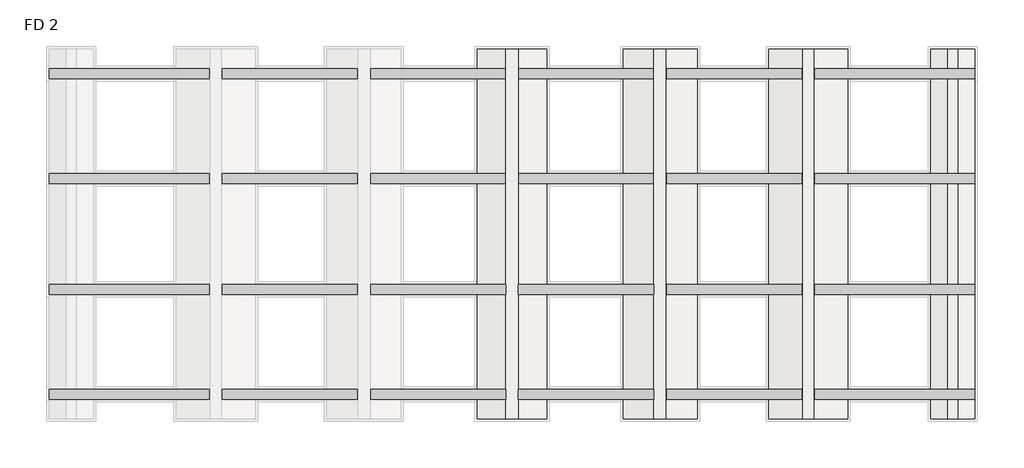
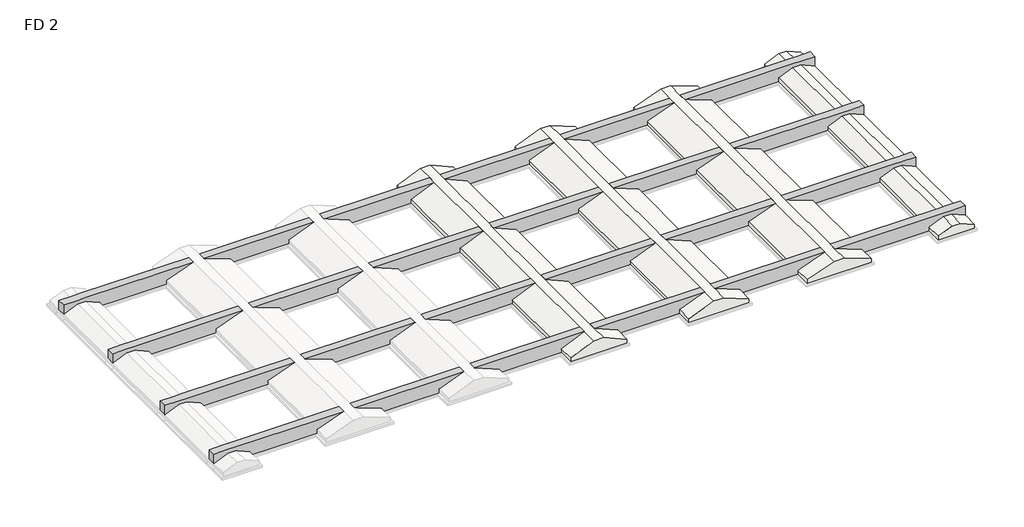
# One storey, part 2 of 2: 4 beams, 4 slabs.
"""IFC4 building model written with IfcOpenShell, lengths in millimetres."""

from ifc_helpers import new_model, si_unit, origin, place, context, project, spatial, faceted_brep, element, save

model = new_model("IFC4")

# Units and contexts
model_context = context("Model", 3, world=origin())
ifc_project = project(units=[si_unit("LENGTHUNIT", "METRE", prefix="MILLI")], contexts=[model_context])

# Site, building, storey
site = spatial("IfcSite", under=ifc_project)
building = spatial("IfcBuilding", under=site)
storey = spatial("IfcBuildingStorey", under=building, Name="FD 2", Elevation=-2170.0)

# Beams
placement = place(None, origin())
element("IfcBeam", 1, ObjectType="M_Concrete-Rectangular Beam : 400x700", at=placement, inside=storey, context=model_context, shape_type="Brep", body=[
    faceted_brep([(-900.0, 12800.0000002, -1470.0), (-900.0, 13200.0000002, -1470.0), (-900.0, 13200.0000002, -1970.0), (-900.0, 12800.0000002, -1970.0), (-200.0, 12800.0000002, -1470.0), (200.0, 12800.0000002, -1470.0), (5600.0000012, 12800.0000002, -1470.0), (5600.0000012, 13200.0000002, -1470.0), (200.0, 13200.0000002, -1470.0), (-200.0, 13200.0000002, -1470.0), (4250.0000012, 13200.0000002, -1970.0), (4250.0000012, 13200.0000002, -2170.0), (900.0, 13200.0000002, -2170.0), (900.0, 13200.0000002, -1970.0), (200.0, 13200.0000002, -1670.0), (-200.0, 13200.0000002, -1670.0), (900.0, 12800.0000002, -2170.0), (4250.0000012, 12800.0000002, -2170.0), (-200.0, 12800.0000002, -1670.0), (200.0, 12800.0000002, -1670.0), (900.0, 12800.0000002, -1970.0), (4250.0000012, 12800.0000002, -1970.0)], [[[0, 1, 2, 3]], [[1, 0, 4, 5, 6, 7, 8, 9]], [[2, 1, 9, 8, 7, 10, 11, 12, 13, 14, 15]], [[16, 12, 11, 17]], [[0, 3, 18, 19, 20, 16, 17, 21, 6, 5, 4]], [[20, 13, 12, 16]], [[13, 20, 19, 14]], [[15, 14, 19, 18]], [[21, 10, 7, 6]], [[10, 21, 17, 11]], [[3, 2, 15, 18]]]),
    faceted_brep([(36599.948043, 13200.0000002, -1470.0), (36599.948043, 12800.0000002, -1470.0), (36599.948043, 12800.0000002, -1970.0), (36599.948043, 13200.0000002, -1970.0), (35899.948043, 12800.0000002, -1670.0), (35899.948043, 13200.0000002, -1670.0), (34799.948043, 13200.0000002, -1970.0), (34799.948043, 12800.0000002, -1970.0), (34799.948043, 12800.0000002, -2170.0), (34799.948043, 13200.0000002, -2170.0), (35499.948043, 13200.0000002, -1670.0), (35499.948043, 12800.0000002, -1670.0), (31449.9130271, 12800.0000002, -1970.0), (31449.9130271, 13200.0000002, -1970.0), (31449.9130271, 13200.0000002, -2170.0), (31449.9130271, 12800.0000002, -2170.0), (30099.9130271, 12800.0000002, -1470.0), (30099.9130271, 13200.0000002, -1470.0), (35899.948043, 13200.0000002, -1470.0), (35499.948043, 13200.0000002, -1470.0), (35499.948043, 12800.0000002, -1470.0), (35899.948043, 12800.0000002, -1470.0)], [[[0, 1, 2, 3]], [[3, 2, 4, 5]], [[6, 7, 8, 9]], [[7, 6, 10, 11]], [[5, 4, 11, 10]], [[12, 13, 14, 15]], [[13, 12, 16, 17]], [[9, 8, 15, 14]], [[1, 0, 18, 19, 17, 16, 20, 21]], [[0, 3, 5, 10, 6, 9, 14, 13, 17, 19, 18]], [[2, 1, 21, 20, 16, 12, 15, 8, 7, 11, 4]]]),
    faceted_brep([(7450.0000012, 12800.0000002, -1970.0), (7450.0000012, 13200.0000002, -1970.0), (7450.0000012, 13200.0000002, -2170.0), (7450.0000012, 12800.0000002, -2170.0), (6100.0000012, 12800.0000002, -1470.0), (6100.0000012, 13200.0000002, -1470.0), (10349.9130239, 13200.0000002, -2170.0), (10349.9130239, 12800.0000002, -2170.0), (10349.9130239, 12800.0000002, -1970.0), (10349.9130239, 13200.0000002, -1970.0), (11599.9130239, 13200.0000002, -1470.0), (11599.9130239, 12800.0000002, -1470.0)], [[[0, 1, 2, 3]], [[1, 0, 4, 5]], [[3, 2, 6, 7]], [[8, 9, 10, 11]], [[9, 8, 7, 6]], [[5, 4, 11, 10]], [[2, 1, 5, 10, 9, 6]], [[3, 7, 8, 11, 4, 0]]]),
    faceted_brep([(13349.9130239, 12800.0000002, -1970.0), (13349.9130239, 13200.0000002, -1970.0), (13349.9130239, 13200.0000002, -2170.0), (13349.9130239, 12800.0000002, -2170.0), (12099.9130239, 12800.0000002, -1470.0), (12099.9130239, 13200.0000002, -1470.0), (16449.7667691, 13200.0000002, -2170.0), (16449.7667691, 12800.0000002, -2170.0), (16449.7667691, 12800.0000002, -1970.0), (16449.7667691, 13200.0000002, -1970.0), (17599.7667691, 13200.0000002, -1470.0), (17599.7667691, 12800.0000002, -1470.0)], [[[0, 1, 2, 3]], [[1, 0, 4, 5]], [[3, 2, 6, 7]], [[8, 9, 10, 11]], [[9, 8, 7, 6]], [[5, 4, 11, 10]], [[2, 1, 5, 10, 9, 6]], [[3, 7, 8, 11, 4, 0]]]),
    faceted_brep([(19249.7667691, 12800.0000002, -1970.0), (19249.7667691, 13200.0000002, -1970.0), (19249.7667691, 13200.0000002, -2170.0), (19249.7667691, 12800.0000002, -2170.0), (18099.7667691, 12800.0000002, -1470.0), (18099.7667691, 13200.0000002, -1470.0), (22349.9130289, 13200.0000002, -2170.0), (22349.9130289, 12800.0000002, -2170.0), (22349.9130289, 12800.0000002, -1970.0), (22349.9130289, 13200.0000002, -1970.0), (23599.9130289, 13200.0000002, -1470.0), (23599.9130289, 12800.0000002, -1470.0)], [[[0, 1, 2, 3]], [[1, 0, 4, 5]], [[3, 2, 6, 7]], [[8, 9, 10, 11]], [[9, 8, 7, 6]], [[5, 4, 11, 10]], [[2, 1, 5, 10, 9, 6]], [[3, 7, 8, 11, 4, 0]]]),
    faceted_brep([(25349.9130289, 12800.0000002, -1970.0), (25349.9130289, 13200.0000002, -1970.0), (25349.9130289, 13200.0000002, -2170.0), (25349.9130289, 12800.0000002, -2170.0), (24099.9130289, 12800.0000002, -1470.0), (24099.9130289, 13200.0000002, -1470.0), (28249.9130271, 13200.0000002, -2170.0), (28249.9130271, 12800.0000002, -2170.0), (28249.9130271, 12800.0000002, -1970.0), (28249.9130271, 13200.0000002, -1970.0), (29599.9130271, 13200.0000002, -1470.0), (29599.9130271, 12800.0000002, -1470.0)], [[[0, 1, 2, 3]], [[1, 0, 4, 5]], [[3, 2, 6, 7]], [[8, 9, 10, 11]], [[9, 8, 7, 6]], [[5, 4, 11, 10]], [[2, 1, 5, 10, 9, 6]], [[0, 3, 7, 8, 11, 4]]]),
])
element("IfcBeam", 2, ObjectType="M_Concrete-Rectangular Beam : 400x700", at=placement, inside=storey, context=model_context, shape_type="Brep", body=[
    faceted_brep([(-900.0, 8550.0000002, -1470.0), (-900.0, 8950.0000002, -1470.0), (-900.0, 8950.0000002, -1970.0), (-900.0, 8550.0000002, -1970.0), (-200.0, 8550.0000002, -1470.0), (200.0, 8550.0000002, -1470.0), (5600.0000012, 8550.0000002, -1470.0), (5600.0000012, 8950.0000002, -1470.0), (200.0, 8950.0000002, -1470.0), (-200.0, 8950.0000002, -1470.0), (4250.0000012, 8950.0000002, -1970.0), (4250.0000012, 8950.0000002, -2170.0), (900.0, 8950.0000002, -2170.0), (900.0, 8950.0000002, -1970.0), (200.0, 8950.0000002, -1670.0), (-200.0, 8950.0000002, -1670.0), (900.0, 8550.0000002, -2170.0), (4250.0000012, 8550.0000002, -2170.0), (-200.0, 8550.0000002, -1670.0), (200.0, 8550.0000002, -1670.0), (900.0, 8550.0000002, -1970.0), (4250.0000012, 8550.0000002, -1970.0)], [[[0, 1, 2, 3]], [[1, 0, 4, 5, 6, 7, 8, 9]], [[2, 1, 9, 8, 7, 10, 11, 12, 13, 14, 15]], [[16, 12, 11, 17]], [[0, 3, 18, 19, 20, 16, 17, 21, 6, 5, 4]], [[3, 2, 15, 18]], [[20, 13, 12, 16]], [[13, 20, 19, 14]], [[15, 14, 19, 18]], [[21, 10, 7, 6]], [[10, 21, 17, 11]]]),
    faceted_brep([(36599.948043, 8950.0000002, -1470.0), (36599.948043, 8550.0000002, -1470.0), (36599.948043, 8550.0000002, -1970.0), (36599.948043, 8950.0000002, -1970.0), (35899.948043, 8550.0000002, -1670.0), (35899.948043, 8950.0000002, -1670.0), (34799.948043, 8950.0000002, -1970.0), (34799.948043, 8550.0000002, -1970.0), (34799.948043, 8550.0000002, -2170.0), (34799.948043, 8950.0000002, -2170.0), (35499.948043, 8950.0000002, -1670.0), (35499.948043, 8550.0000002, -1670.0), (31449.9130271, 8550.0000002, -1970.0), (31449.9130271, 8950.0000002, -1970.0), (31449.9130271, 8950.0000002, -2170.0), (31449.9130271, 8550.0000002, -2170.0), (30099.9130271, 8550.0000002, -1470.0), (30099.9130271, 8950.0000002, -1470.0), (35899.948043, 8950.0000002, -1470.0), (35499.948043, 8950.0000002, -1470.0), (35499.948043, 8550.0000002, -1470.0), (35899.948043, 8550.0000002, -1470.0)], [[[0, 1, 2, 3]], [[3, 2, 4, 5]], [[6, 7, 8, 9]], [[7, 6, 10, 11]], [[5, 4, 11, 10]], [[12, 13, 14, 15]], [[13, 12, 16, 17]], [[9, 8, 15, 14]], [[1, 0, 18, 19, 17, 16, 20, 21]], [[0, 3, 5, 10, 6, 9, 14, 13, 17, 19, 18]], [[2, 1, 21, 20, 16, 12, 15, 8, 7, 11, 4]]]),
    faceted_brep([(7450.0000012, 8550.0000002, -1970.0), (7450.0000012, 8950.0000002, -1970.0), (7450.0000012, 8950.0000002, -2170.0), (7450.0000012, 8550.0000002, -2170.0), (6100.0000012, 8550.0000002, -1470.0), (6100.0000012, 8950.0000002, -1470.0), (10349.9130239, 8950.0000002, -2170.0), (10349.9130239, 8550.0000002, -2170.0), (10349.9130239, 8550.0000002, -1970.0), (10349.9130239, 8950.0000002, -1970.0), (11599.9130239, 8950.0000002, -1470.0), (11599.9130239, 8550.0000002, -1470.0)], [[[0, 1, 2, 3]], [[1, 0, 4, 5]], [[3, 2, 6, 7]], [[8, 9, 10, 11]], [[9, 8, 7, 6]], [[5, 4, 11, 10]], [[2, 1, 5, 10, 9, 6]], [[3, 7, 8, 11, 4, 0]]]),
    faceted_brep([(13349.9130239, 8550.0000002, -1970.0), (13349.9130239, 8950.0000002, -1970.0), (13349.9130239, 8950.0000002, -2170.0), (13349.9130239, 8550.0000002, -2170.0), (12099.9130239, 8550.0000002, -1470.0), (12099.9130239, 8950.0000002, -1470.0), (16449.7667691, 8950.0000002, -2170.0), (16449.7667691, 8550.0000002, -2170.0), (16449.7667691, 8550.0000002, -1970.0), (16449.7667691, 8950.0000002, -1970.0), (17599.7667691, 8950.0000002, -1470.0), (17599.7667691, 8550.0000002, -1470.0)], [[[0, 1, 2, 3]], [[1, 0, 4, 5]], [[3, 2, 6, 7]], [[8, 9, 10, 11]], [[9, 8, 7, 6]], [[5, 4, 11, 10]], [[2, 1, 5, 10, 9, 6]], [[3, 7, 8, 11, 4, 0]]]),
    faceted_brep([(19249.7667691, 8550.0000002, -1970.0), (19249.7667691, 8950.0000002, -1970.0), (19249.7667691, 8950.0000002, -2170.0), (19249.7667691, 8550.0000002, -2170.0), (18099.7667691, 8550.0000002, -1470.0), (18099.7667691, 8950.0000002, -1470.0), (22349.9130289, 8950.0000002, -2170.0), (22349.9130289, 8550.0000002, -2170.0), (22349.9130289, 8550.0000002, -1970.0), (22349.9130289, 8950.0000002, -1970.0), (23599.9130289, 8950.0000002, -1470.0), (23599.9130289, 8550.0000002, -1470.0)], [[[0, 1, 2, 3]], [[1, 0, 4, 5]], [[3, 2, 6, 7]], [[8, 9, 10, 11]], [[9, 8, 7, 6]], [[5, 4, 11, 10]], [[2, 1, 5, 10, 9, 6]], [[3, 7, 8, 11, 4, 0]]]),
    faceted_brep([(25349.9130289, 8550.0000002, -1970.0), (25349.9130289, 8950.0000002, -1970.0), (25349.9130289, 8950.0000002, -2170.0), (25349.9130289, 8550.0000002, -2170.0), (24099.9130289, 8550.0000002, -1470.0), (24099.9130289, 8950.0000002, -1470.0), (28249.9130271, 8950.0000002, -2170.0), (28249.9130271, 8550.0000002, -2170.0), (28249.9130271, 8550.0000002, -1970.0), (28249.9130271, 8950.0000002, -1970.0), (29599.9130271, 8950.0000002, -1470.0), (29599.9130271, 8550.0000002, -1470.0)], [[[0, 1, 2, 3]], [[1, 0, 4, 5]], [[3, 2, 6, 7]], [[8, 9, 10, 11]], [[9, 8, 7, 6]], [[5, 4, 11, 10]], [[2, 1, 5, 10, 9, 6]], [[0, 3, 7, 8, 11, 4]]]),
])
element("IfcBeam", 3, ObjectType="M_Concrete-Rectangular Beam : 400x700", at=placement, inside=storey, context=model_context, shape_type="Brep", body=[
    faceted_brep([(-900.0, 4050.0000002, -1470.0), (-900.0, 4450.0000002, -1470.0), (-900.0, 4450.0000002, -1970.0), (-900.0, 4050.0000002, -1970.0), (-200.0, 4050.0000002, -1470.0), (200.0, 4050.0000002, -1470.0), (5600.0000012, 4050.0000002, -1470.0), (5600.0000012, 4450.0000002, -1470.0), (200.0, 4450.0000002, -1470.0), (-200.0, 4450.0000002, -1470.0), (4250.0000012, 4450.0000002, -1970.0), (4250.0000012, 4450.0000002, -2170.0), (900.0, 4450.0000002, -2170.0), (900.0, 4450.0000002, -1970.0), (200.0, 4450.0000002, -1670.0), (-200.0, 4450.0000002, -1670.0), (900.0, 4050.0000002, -2170.0), (4250.0000012, 4050.0000002, -2170.0), (-200.0, 4050.0000002, -1670.0), (200.0, 4050.0000002, -1670.0), (900.0, 4050.0000002, -1970.0), (4250.0000012, 4050.0000002, -1970.0)], [[[0, 1, 2, 3]], [[1, 0, 4, 5, 6, 7, 8, 9]], [[2, 1, 9, 8, 7, 10, 11, 12, 13, 14, 15]], [[16, 12, 11, 17]], [[0, 3, 18, 19, 20, 16, 17, 21, 6, 5, 4]], [[3, 2, 15, 18]], [[20, 13, 12, 16]], [[13, 20, 19, 14]], [[15, 14, 19, 18]], [[21, 10, 7, 6]], [[10, 21, 17, 11]]]),
    faceted_brep([(36599.948043, 4450.0000002, -1470.0), (36599.948043, 4050.0000002, -1470.0), (36599.948043, 4050.0000002, -1970.0), (36599.948043, 4450.0000002, -1970.0), (35899.948043, 4050.0000002, -1670.0), (35899.948043, 4450.0000002, -1670.0), (34799.948043, 4450.0000002, -1970.0), (34799.948043, 4050.0000002, -1970.0), (34799.948043, 4050.0000002, -2170.0), (34799.948043, 4450.0000002, -2170.0), (35499.948043, 4450.0000002, -1670.0), (35499.948043, 4050.0000002, -1670.0), (31449.9130271, 4050.0000002, -1970.0), (31449.9130271, 4450.0000002, -1970.0), (31449.9130271, 4450.0000002, -2170.0), (31449.9130271, 4050.0000002, -2170.0), (30099.9130271, 4050.0000002, -1470.0), (30099.9130271, 4450.0000002, -1470.0), (35899.948043, 4450.0000002, -1470.0), (35499.948043, 4450.0000002, -1470.0), (35499.948043, 4050.0000002, -1470.0), (35899.948043, 4050.0000002, -1470.0)], [[[0, 1, 2, 3]], [[3, 2, 4, 5]], [[6, 7, 8, 9]], [[7, 6, 10, 11]], [[5, 4, 11, 10]], [[12, 13, 14, 15]], [[13, 12, 16, 17]], [[9, 8, 15, 14]], [[1, 0, 18, 19, 17, 16, 20, 21]], [[0, 3, 5, 10, 6, 9, 14, 13, 17, 19, 18]], [[2, 1, 21, 20, 16, 12, 15, 8, 7, 11, 4]]]),
    faceted_brep([(7450.0000012, 4050.0000002, -1970.0), (7450.0000012, 4450.0000002, -1970.0), (7450.0000012, 4450.0000002, -2170.0), (7450.0000012, 4050.0000002, -2170.0), (6100.0000012, 4050.0000002, -1470.0), (6100.0000012, 4450.0000002, -1470.0), (10349.9130239, 4450.0000002, -2170.0), (10349.9130239, 4050.0000002, -2170.0), (10349.9130239, 4050.0000002, -1970.0), (10349.9130239, 4450.0000002, -1970.0), (11599.9130239, 4450.0000002, -1470.0), (11599.9130239, 4050.0000002, -1470.0)], [[[0, 1, 2, 3]], [[1, 0, 4, 5]], [[3, 2, 6, 7]], [[8, 9, 10, 11]], [[9, 8, 7, 6]], [[5, 4, 11, 10]], [[2, 1, 5, 10, 9, 6]], [[3, 7, 8, 11, 4, 0]]]),
    faceted_brep([(13349.9130239, 4050.0000002, -1970.0), (13349.9130239, 4450.0000002, -1970.0), (13349.9130239, 4450.0000002, -2170.0), (13349.9130239, 4050.0000002, -2170.0), (12099.9130239, 4050.0000002, -1470.0), (12099.9130239, 4450.0000002, -1470.0), (16449.7667691, 4450.0000002, -2170.0), (16449.7667691, 4050.0000002, -2170.0), (16449.7667691, 4050.0000002, -1970.0), (16449.7667691, 4450.0000002, -1970.0), (17599.7667691, 4450.0000002, -1470.0), (17599.7667691, 4050.0000002, -1470.0)], [[[0, 1, 2, 3]], [[1, 0, 4, 5]], [[3, 2, 6, 7]], [[8, 9, 10, 11]], [[9, 8, 7, 6]], [[5, 4, 11, 10]], [[2, 1, 5, 10, 9, 6]], [[3, 7, 8, 11, 4, 0]]]),
    faceted_brep([(19249.7667691, 4050.0000002, -1970.0), (19249.7667691, 4450.0000002, -1970.0), (19249.7667691, 4450.0000002, -2170.0), (19249.7667691, 4050.0000002, -2170.0), (18099.7667691, 4050.0000002, -1470.0), (18099.7667691, 4450.0000002, -1470.0), (22349.9130289, 4450.0000002, -2170.0), (22349.9130289, 4050.0000002, -2170.0), (22349.9130289, 4050.0000002, -1970.0), (22349.9130289, 4450.0000002, -1970.0), (23599.9130289, 4450.0000002, -1470.0), (23599.9130289, 4050.0000002, -1470.0)], [[[0, 1, 2, 3]], [[1, 0, 4, 5]], [[3, 2, 6, 7]], [[8, 9, 10, 11]], [[9, 8, 7, 6]], [[5, 4, 11, 10]], [[2, 1, 5, 10, 9, 6]], [[3, 7, 8, 11, 4, 0]]]),
    faceted_brep([(25349.9130289, 4050.0000002, -1970.0), (25349.9130289, 4450.0000002, -1970.0), (25349.9130289, 4450.0000002, -2170.0), (25349.9130289, 4050.0000002, -2170.0), (24099.9130289, 4050.0000002, -1470.0), (24099.9130289, 4450.0000002, -1470.0), (28249.9130271, 4450.0000002, -2170.0), (28249.9130271, 4050.0000002, -2170.0), (28249.9130271, 4050.0000002, -1970.0), (28249.9130271, 4450.0000002, -1970.0), (29599.9130271, 4450.0000002, -1470.0), (29599.9130271, 4050.0000002, -1470.0)], [[[0, 1, 2, 3]], [[1, 0, 4, 5]], [[3, 2, 6, 7]], [[8, 9, 10, 11]], [[9, 8, 7, 6]], [[5, 4, 11, 10]], [[2, 1, 5, 10, 9, 6]], [[0, 3, 7, 8, 11, 4]]]),
])
element("IfcBeam", 4, ObjectType="M_Concrete-Rectangular Beam : 400x700", at=placement, inside=storey, context=model_context, shape_type="Brep", body=[
    faceted_brep([(-900.0, -200.0, -1470.0), (-900.0, 200.0, -1470.0), (-900.0, 200.0, -1970.0), (-900.0, -200.0, -1970.0), (-200.0, -200.0, -1470.0), (200.0, -200.0, -1470.0), (5600.0000012, -200.0, -1470.0), (5600.0000012, 200.0, -1470.0), (200.0, 200.0, -1470.0), (-200.0, 200.0, -1470.0), (4250.0000012, 200.0, -1970.0), (4250.0000012, 200.0, -2170.0), (900.0, 200.0, -2170.0), (900.0, 200.0, -1970.0), (200.0, 200.0, -1670.0), (-200.0, 200.0, -1670.0), (900.0, -200.0, -2170.0), (4250.0000012, -200.0, -2170.0), (-200.0, -200.0, -1670.0), (200.0, -200.0, -1670.0), (900.0, -200.0, -1970.0), (4250.0000012, -200.0, -1970.0)], [[[0, 1, 2, 3]], [[1, 0, 4, 5, 6, 7, 8, 9]], [[2, 1, 9, 8, 7, 10, 11, 12, 13, 14, 15]], [[16, 12, 11, 17]], [[0, 3, 18, 19, 20, 16, 17, 21, 6, 5, 4]], [[3, 2, 15, 18]], [[20, 13, 12, 16]], [[13, 20, 19, 14]], [[15, 14, 19, 18]], [[21, 10, 7, 6]], [[10, 21, 17, 11]]]),
    faceted_brep([(36599.948043, 200.0, -1470.0), (36599.948043, -200.0, -1470.0), (36599.948043, -200.0, -1970.0), (36599.948043, 200.0, -1970.0), (35899.948043, -200.0, -1670.0), (35899.948043, 200.0, -1670.0), (34799.948043, 200.0, -1970.0), (34799.948043, -200.0, -1970.0), (34799.948043, -200.0, -2170.0), (34799.948043, 200.0, -2170.0), (35499.948043, 200.0, -1670.0), (35499.948043, -200.0, -1670.0), (31449.9130271, -200.0, -1970.0), (31449.9130271, 200.0, -1970.0), (31449.9130271, 200.0, -2170.0), (31449.9130271, -200.0, -2170.0), (30099.9130271, -200.0, -1470.0), (30099.9130271, 200.0, -1470.0), (35899.948043, 200.0, -1470.0), (35499.948043, 200.0, -1470.0), (35499.948043, -200.0, -1470.0), (35899.948043, -200.0, -1470.0)], [[[0, 1, 2, 3]], [[3, 2, 4, 5]], [[6, 7, 8, 9]], [[7, 6, 10, 11]], [[5, 4, 11, 10]], [[12, 13, 14, 15]], [[13, 12, 16, 17]], [[9, 8, 15, 14]], [[1, 0, 18, 19, 17, 16, 20, 21]], [[0, 3, 5, 10, 6, 9, 14, 13, 17, 19, 18]], [[2, 1, 21, 20, 16, 12, 15, 8, 7, 11, 4]]]),
    faceted_brep([(7450.0000012, -200.0, -1970.0), (7450.0000012, 200.0, -1970.0), (7450.0000012, 200.0, -2170.0), (7450.0000012, -200.0, -2170.0), (6100.0000012, -200.0, -1470.0), (6100.0000012, 200.0, -1470.0), (10349.9130239, 200.0, -2170.0), (10349.9130239, -200.0, -2170.0), (10349.9130239, -200.0, -1970.0), (10349.9130239, 200.0, -1970.0), (11599.9130239, 200.0, -1470.0), (11599.9130239, -200.0, -1470.0)], [[[0, 1, 2, 3]], [[1, 0, 4, 5]], [[3, 2, 6, 7]], [[8, 9, 10, 11]], [[9, 8, 7, 6]], [[5, 4, 11, 10]], [[2, 1, 5, 10, 9, 6]], [[3, 7, 8, 11, 4, 0]]]),
    faceted_brep([(13349.9130239, -200.0, -1970.0), (13349.9130239, 200.0, -1970.0), (13349.9130239, 200.0, -2170.0), (13349.9130239, -200.0, -2170.0), (12099.9130239, -200.0, -1470.0), (12099.9130239, 200.0, -1470.0), (16449.7667691, 200.0, -2170.0), (16449.7667691, -200.0, -2170.0), (16449.7667691, -200.0, -1970.0), (16449.7667691, 200.0, -1970.0), (17599.7667691, 200.0, -1470.0), (17599.7667691, -200.0, -1470.0)], [[[0, 1, 2, 3]], [[1, 0, 4, 5]], [[3, 2, 6, 7]], [[8, 9, 10, 11]], [[9, 8, 7, 6]], [[5, 4, 11, 10]], [[2, 1, 5, 10, 9, 6]], [[3, 7, 8, 11, 4, 0]]]),
    faceted_brep([(19249.7667691, -200.0, -1970.0), (19249.7667691, 200.0, -1970.0), (19249.7667691, 200.0, -2170.0), (19249.7667691, -200.0, -2170.0), (18099.7667691, -200.0, -1470.0), (18099.7667691, 200.0, -1470.0), (22349.9130289, 200.0, -2170.0), (22349.9130289, -200.0, -2170.0), (22349.9130289, -200.0, -1970.0), (22349.9130289, 200.0, -1970.0), (23599.9130289, 200.0, -1470.0), (23599.9130289, -200.0, -1470.0)], [[[0, 1, 2, 3]], [[1, 0, 4, 5]], [[3, 2, 6, 7]], [[8, 9, 10, 11]], [[9, 8, 7, 6]], [[5, 4, 11, 10]], [[2, 1, 5, 10, 9, 6]], [[3, 7, 8, 11, 4, 0]]]),
    faceted_brep([(25349.9130289, -200.0, -1970.0), (25349.9130289, 200.0, -1970.0), (25349.9130289, 200.0, -2170.0), (25349.9130289, -200.0, -2170.0), (24099.9130289, -200.0, -1470.0), (24099.9130289, 200.0, -1470.0), (28249.9130271, 200.0, -2170.0), (28249.9130271, -200.0, -2170.0), (28249.9130271, -200.0, -1970.0), (28249.9130271, 200.0, -1970.0), (29599.9130271, 200.0, -1470.0), (29599.9130271, -200.0, -1470.0)], [[[0, 1, 2, 3]], [[1, 0, 4, 5]], [[3, 2, 6, 7]], [[8, 9, 10, 11]], [[9, 8, 7, 6]], [[5, 4, 11, 10]], [[2, 1, 5, 10, 9, 6]], [[0, 3, 7, 8, 11, 4]]]),
])

# Slabs
element("IfcSlab", 5, ObjectType="Mong bang-lech tam : 1800x700", at=placement, inside=storey, context=model_context, shape_type="Brep", body=[
    faceted_brep([(35899.948043, -999.9999998, -1670.0), (35499.948043, -999.9999998, -1670.0), (34799.948043, -999.9999998, -1970.0), (34799.948043, -999.9999998, -2170.0), (36599.948043, -999.9999998, -2170.0), (36599.948043, -999.9999998, -1970.0), (35899.948043, 14000.0000002, -1670.0), (36599.948043, 14000.0000002, -1970.0), (36599.948043, 14000.0000002, -2170.0), (34799.948043, 14000.0000002, -2170.0), (34799.948043, 14000.0000002, -1970.0), (35499.948043, 14000.0000002, -1670.0), (36599.948043, -200.0, -1970.0), (36599.948043, 200.0, -1970.0), (36599.948043, 4050.0000002, -1970.0), (36599.948043, 4450.0000002, -1970.0), (36599.948043, 8550.0000002, -1970.0), (36599.948043, 8950.0000002, -1970.0), (36599.948043, 12800.0000002, -1970.0), (36599.948043, 13200.0000002, -1970.0), (35899.948043, 13200.0000002, -1670.0), (35899.948043, 12800.0000002, -1670.0), (35899.948043, 8950.0000002, -1670.0), (35899.948043, 8550.0000002, -1670.0), (35899.948043, 4450.0000002, -1670.0), (35899.948043, 4050.0000002, -1670.0), (35899.948043, 200.0, -1670.0), (35899.948043, -200.0, -1670.0), (34799.948043, -200.0, -2170.0), (34799.948043, 200.0, -2170.0), (34799.948043, 4050.0000002, -2170.0), (34799.948043, 4450.0000002, -2170.0), (34799.948043, 8550.0000002, -2170.0), (34799.948043, 8950.0000002, -2170.0), (34799.948043, 12800.0000002, -2170.0), (34799.948043, 13200.0000002, -2170.0), (34799.948043, -200.0, -1970.0), (34799.948043, 200.0, -1970.0), (34799.948043, 4050.0000002, -1970.0), (34799.948043, 4450.0000002, -1970.0), (34799.948043, 8550.0000002, -1970.0), (34799.948043, 8950.0000002, -1970.0), (34799.948043, 12800.0000002, -1970.0), (34799.948043, 13200.0000002, -1970.0), (35499.948043, -200.0, -1670.0), (35499.948043, 200.0, -1670.0), (35499.948043, 4050.0000002, -1670.0), (35499.948043, 4450.0000002, -1670.0), (35499.948043, 8550.0000002, -1670.0), (35499.948043, 8950.0000002, -1670.0), (35499.948043, 12800.0000002, -1670.0), (35499.948043, 13200.0000002, -1670.0)], [[[0, 1, 2, 3, 4, 5]], [[6, 7, 8, 9, 10, 11]], [[5, 12, 13, 14, 15, 16, 17, 18, 19, 7, 6, 20, 21, 22, 23, 24, 25, 26, 27, 0]], [[4, 8, 7, 19, 18, 17, 16, 15, 14, 13, 12, 5]], [[3, 28, 29, 30, 31, 32, 33, 34, 35, 9, 8, 4]], [[2, 36, 37, 38, 39, 40, 41, 42, 43, 10, 9, 35, 34, 33, 32, 31, 30, 29, 28, 3]], [[1, 44, 45, 46, 47, 48, 49, 50, 51, 11, 10, 43, 42, 41, 40, 39, 38, 37, 36, 2]], [[0, 27, 26, 25, 24, 23, 22, 21, 20, 6, 11, 51, 50, 49, 48, 47, 46, 45, 44, 1]]]),
])
element("IfcSlab", 6, ObjectType="Mong bang-lech tam : 2800x1000", at=placement, inside=storey, context=model_context, shape_type="Brep", body=[
    faceted_brep([(17599.7667691, -999.9999998, -1470.0), (16449.7667691, -999.9999998, -1970.0), (16449.7667691, -999.9999998, -2170.0), (19249.7667691, -999.9999998, -2170.0), (19249.7667691, -999.9999998, -1970.0), (18099.7667691, -999.9999998, -1470.0), (17599.7667691, 14000.0000002, -1470.0), (18099.7667691, 14000.0000002, -1470.0), (19249.7667691, 14000.0000002, -1970.0), (19249.7667691, 14000.0000002, -2170.0), (16449.7667691, 14000.0000002, -2170.0), (16449.7667691, 14000.0000002, -1970.0), (17599.7667691, -200.0, -1470.0), (17599.7667691, 200.0, -1470.0), (17599.7667691, 4050.0000002, -1470.0), (17599.7667691, 4450.0000002, -1470.0), (17599.7667691, 8550.0000002, -1470.0), (17599.7667691, 8950.0000002, -1470.0), (17599.7667691, 12800.0000002, -1470.0), (17599.7667691, 13200.0000002, -1470.0), (16449.7667691, 13200.0000002, -1970.0), (16449.7667691, 12800.0000002, -1970.0), (16449.7667691, 8950.0000002, -1970.0), (16449.7667691, 8550.0000002, -1970.0), (16449.7667691, 4450.0000002, -1970.0), (16449.7667691, 4050.0000002, -1970.0), (16449.7667691, 200.0, -1970.0), (16449.7667691, -200.0, -1970.0), (16449.7667691, 13200.0000002, -2170.0), (16449.7667691, 12800.0000002, -2170.0), (16449.7667691, 8950.0000002, -2170.0), (16449.7667691, 8550.0000002, -2170.0), (16449.7667691, 4450.0000002, -2170.0), (16449.7667691, 4050.0000002, -2170.0), (16449.7667691, 200.0, -2170.0), (16449.7667691, -200.0, -2170.0), (19249.7667691, 13200.0000002, -2170.0), (19249.7667691, 12800.0000002, -2170.0), (19249.7667691, 8950.0000002, -2170.0), (19249.7667691, 8550.0000002, -2170.0), (19249.7667691, 4450.0000002, -2170.0), (19249.7667691, 4050.0000002, -2170.0), (19249.7667691, 200.0, -2170.0), (19249.7667691, -200.0, -2170.0), (19249.7667691, 13200.0000002, -1970.0), (19249.7667691, 12800.0000002, -1970.0), (19249.7667691, 8950.0000002, -1970.0), (19249.7667691, 8550.0000002, -1970.0), (19249.7667691, 4450.0000002, -1970.0), (19249.7667691, 4050.0000002, -1970.0), (19249.7667691, 200.0, -1970.0), (19249.7667691, -200.0, -1970.0), (18099.7667691, 13200.0000002, -1470.0), (18099.7667691, 12800.0000002, -1470.0), (18099.7667691, 8950.0000002, -1470.0), (18099.7667691, 8550.0000002, -1470.0), (18099.7667691, 4450.0000002, -1470.0), (18099.7667691, 4050.0000002, -1470.0), (18099.7667691, 200.0, -1470.0), (18099.7667691, -200.0, -1470.0)], [[[0, 1, 2, 3, 4, 5]], [[6, 7, 8, 9, 10, 11]], [[1, 0, 12, 13, 14, 15, 16, 17, 18, 19, 6, 11, 20, 21, 22, 23, 24, 25, 26, 27]], [[2, 1, 27, 26, 25, 24, 23, 22, 21, 20, 11, 10, 28, 29, 30, 31, 32, 33, 34, 35]], [[3, 2, 35, 34, 33, 32, 31, 30, 29, 28, 10, 9, 36, 37, 38, 39, 40, 41, 42, 43]], [[4, 3, 43, 42, 41, 40, 39, 38, 37, 36, 9, 8, 44, 45, 46, 47, 48, 49, 50, 51]], [[5, 4, 51, 50, 49, 48, 47, 46, 45, 44, 8, 7, 52, 53, 54, 55, 56, 57, 58, 59]], [[0, 5, 59, 58, 57, 56, 55, 54, 53, 52, 7, 6, 19, 18, 17, 16, 15, 14, 13, 12]]]),
])
element("IfcSlab", 7, ObjectType="Mong bang-lech tam : 3000x1000", at=placement, inside=storey, context=model_context, shape_type="Brep", body=[
    faceted_brep([(23599.9130289, -999.9999998, -1470.0), (22349.9130289, -999.9999998, -1970.0), (22349.9130289, -999.9999998, -2170.0), (25349.9130289, -999.9999998, -2170.0), (25349.9130289, -999.9999998, -1970.0), (24099.9130289, -999.9999998, -1470.0), (23599.9130289, 14000.0000002, -1470.0), (24099.9130289, 14000.0000002, -1470.0), (25349.9130289, 14000.0000002, -1970.0), (25349.9130289, 14000.0000002, -2170.0), (22349.9130289, 14000.0000002, -2170.0), (22349.9130289, 14000.0000002, -1970.0), (23599.9130289, -200.0, -1470.0), (23599.9130289, 200.0, -1470.0), (23599.9130289, 4050.0000002, -1470.0), (23599.9130289, 4450.0000002, -1470.0), (23599.9130289, 8550.0000002, -1470.0), (23599.9130289, 8950.0000002, -1470.0), (23599.9130289, 12800.0000002, -1470.0), (23599.9130289, 13200.0000002, -1470.0), (22349.9130289, 13200.0000002, -1970.0), (22349.9130289, 12800.0000002, -1970.0), (22349.9130289, 8950.0000002, -1970.0), (22349.9130289, 8550.0000002, -1970.0), (22349.9130289, 4450.0000002, -1970.0), (22349.9130289, 4050.0000002, -1970.0), (22349.9130289, 200.0, -1970.0), (22349.9130289, -200.0, -1970.0), (22349.9130289, 13200.0000002, -2170.0), (22349.9130289, 12800.0000002, -2170.0), (22349.9130289, 8950.0000002, -2170.0), (22349.9130289, 8550.0000002, -2170.0), (22349.9130289, 4450.0000002, -2170.0), (22349.9130289, 4050.0000002, -2170.0), (22349.9130289, 200.0, -2170.0), (22349.9130289, -200.0, -2170.0), (25349.9130289, 13200.0000002, -2170.0), (25349.9130289, 12800.0000002, -2170.0), (25349.9130289, 8950.0000002, -2170.0), (25349.9130289, 8550.0000002, -2170.0), (25349.9130289, 4450.0000002, -2170.0), (25349.9130289, 4050.0000002, -2170.0), (25349.9130289, 200.0, -2170.0), (25349.9130289, -200.0, -2170.0), (25349.9130289, 13200.0000002, -1970.0), (25349.9130289, 12800.0000002, -1970.0), (25349.9130289, 8950.0000002, -1970.0), (25349.9130289, 8550.0000002, -1970.0), (25349.9130289, 4450.0000002, -1970.0), (25349.9130289, 4050.0000002, -1970.0), (25349.9130289, 200.0, -1970.0), (25349.9130289, -200.0, -1970.0), (24099.9130289, 13200.0000002, -1470.0), (24099.9130289, 12800.0000002, -1470.0), (24099.9130289, 8950.0000002, -1470.0), (24099.9130289, 8550.0000002, -1470.0), (24099.9130289, 4450.0000002, -1470.0), (24099.9130289, 4050.0000002, -1470.0), (24099.9130289, 200.0, -1470.0), (24099.9130289, -200.0, -1470.0)], [[[0, 1, 2, 3, 4, 5]], [[6, 7, 8, 9, 10, 11]], [[1, 0, 12, 13, 14, 15, 16, 17, 18, 19, 6, 11, 20, 21, 22, 23, 24, 25, 26, 27]], [[2, 1, 27, 26, 25, 24, 23, 22, 21, 20, 11, 10, 28, 29, 30, 31, 32, 33, 34, 35]], [[3, 2, 35, 34, 33, 32, 31, 30, 29, 28, 10, 9, 36, 37, 38, 39, 40, 41, 42, 43]], [[4, 3, 43, 42, 41, 40, 39, 38, 37, 36, 9, 8, 44, 45, 46, 47, 48, 49, 50, 51]], [[5, 4, 51, 50, 49, 48, 47, 46, 45, 44, 8, 7, 52, 53, 54, 55, 56, 57, 58, 59]], [[0, 5, 59, 58, 57, 56, 55, 54, 53, 52, 7, 6, 19, 18, 17, 16, 15, 14, 13, 12]]]),
])
element("IfcSlab", 8, ObjectType="Mong bang-lech tam : 3200x1000", at=placement, inside=storey, context=model_context, shape_type="Brep", body=[
    faceted_brep([(29599.9130271, -999.9999998, -1470.0), (28249.9130271, -999.9999998, -1970.0), (28249.9130271, -999.9999998, -2170.0), (31449.9130271, -999.9999998, -2170.0), (31449.9130271, -999.9999998, -1970.0), (30099.9130271, -999.9999998, -1470.0), (31449.9130271, -200.0, -2170.0), (31449.9130271, 200.0, -2170.0), (31449.9130271, 4050.0000002, -2170.0), (31449.9130271, 4450.0000002, -2170.0), (31449.9130271, 8550.0000002, -2170.0), (31449.9130271, 8950.0000002, -2170.0), (31449.9130271, 12800.0000002, -2170.0), (31449.9130271, 13200.0000002, -2170.0), (31449.9130271, 14000.0000002, -2170.0), (31449.9130271, 14000.0000002, -1970.0), (31449.9130271, 13200.0000002, -1970.0), (31449.9130271, 12800.0000002, -1970.0), (31449.9130271, 8950.0000002, -1970.0), (31449.9130271, 8550.0000002, -1970.0), (31449.9130271, 4450.0000002, -1970.0), (31449.9130271, 4050.0000002, -1970.0), (31449.9130271, 200.0, -1970.0), (31449.9130271, -200.0, -1970.0), (30099.9130271, 14000.0000002, -1470.0), (30099.9130271, 13200.0000002, -1470.0), (30099.9130271, 12800.0000002, -1470.0), (30099.9130271, 8950.0000002, -1470.0), (30099.9130271, 8550.0000002, -1470.0), (30099.9130271, 4450.0000002, -1470.0), (30099.9130271, 4050.0000002, -1470.0), (30099.9130271, 200.0, -1470.0), (30099.9130271, -200.0, -1470.0), (29599.9130271, 14000.0000002, -1470.0), (29599.9130271, 13200.0000002, -1470.0), (29599.9130271, 12800.0000002, -1470.0), (29599.9130271, 8950.0000002, -1470.0), (29599.9130271, 8550.0000002, -1470.0), (29599.9130271, 4450.0000002, -1470.0), (29599.9130271, 4050.0000002, -1470.0), (29599.9130271, 200.0, -1470.0), (29599.9130271, -200.0, -1470.0), (28249.9130271, 14000.0000002, -2170.0), (28249.9130271, 14000.0000002, -1970.0), (28249.9130271, 13200.0000002, -1970.0), (28249.9130271, 12800.0000002, -1970.0), (28249.9130271, 8950.0000002, -1970.0), (28249.9130271, 8550.0000002, -1970.0), (28249.9130271, 4450.0000002, -1970.0), (28249.9130271, 4050.0000002, -1970.0), (28249.9130271, 200.0, -1970.0), (28249.9130271, -200.0, -1970.0), (28249.9130271, 13200.0000002, -2170.0), (28249.9130271, 12800.0000002, -2170.0), (28249.9130271, 8950.0000002, -2170.0), (28249.9130271, 8550.0000002, -2170.0), (28249.9130271, 4450.0000002, -2170.0), (28249.9130271, 4050.0000002, -2170.0), (28249.9130271, 200.0, -2170.0), (28249.9130271, -200.0, -2170.0)], [[[0, 1, 2, 3, 4, 5]], [[4, 3, 6, 7, 8, 9, 10, 11, 12, 13, 14, 15, 16, 17, 18, 19, 20, 21, 22, 23]], [[5, 4, 23, 22, 21, 20, 19, 18, 17, 16, 15, 24, 25, 26, 27, 28, 29, 30, 31, 32]], [[0, 5, 32, 31, 30, 29, 28, 27, 26, 25, 24, 33, 34, 35, 36, 37, 38, 39, 40, 41]], [[33, 24, 15, 14, 42, 43]], [[1, 0, 41, 40, 39, 38, 37, 36, 35, 34, 33, 43, 44, 45, 46, 47, 48, 49, 50, 51]], [[2, 1, 51, 50, 49, 48, 47, 46, 45, 44, 43, 42, 52, 53, 54, 55, 56, 57, 58, 59]], [[3, 2, 59, 58, 57, 56, 55, 54, 53, 52, 42, 14, 13, 12, 11, 10, 9, 8, 7, 6]]]),
])

save(model, "model.ifc")

# Revit data of these elements
# Type "M_Concrete-Rectangular Beam : 400x700"
#   Length [instance default] = 1524 mm
#   b = 400 mm
#   h = 700 mm
#   Structural Material [instance default] = Concrete, Cast-in-Place gray
#   Assembly Code = ""
# Type "Mong bang-lech tam : 1800x700"
#   Length = 15000 mm
#   Lech Tam (E) = 0 mm
#   Foundation Thickness = 500 mm
#   Foundation (h2) = 200 mm
#   Foundation (h1) = 300 mm
#   Be Rong Dam (b) = 400 mm
#   Be Rong Dai Mong (B) = 1800 mm
#   Structural Material [instance default] = Concrete, Cast-in-Place gray
#   Width = 0
#   Assembly Code = ""
# Type "Mong bang-lech tam : 2800x1000"
#   Length = 15000 mm
#   Lech Tam (E) = 0 mm
#   Foundation Thickness = 700 mm
#   Foundation (h2) = 200 mm
#   Foundation (h1) = 500 mm
#   Be Rong Dam (b) = 500 mm
#   Be Rong Dai Mong (B) = 2800 mm
#   Structural Material [instance default] = Concrete, Cast-in-Place gray
#   Width = 0
#   Assembly Code = ""
# Type "Mong bang-lech tam : 3000x1000"
#   Length = 15000 mm
#   Lech Tam (E) = 0 mm
#   Foundation Thickness = 700 mm
#   Foundation (h2) = 200 mm
#   Foundation (h1) = 500 mm
#   Be Rong Dam (b) = 500 mm
#   Be Rong Dai Mong (B) = 3000 mm
#   Structural Material [instance default] = Concrete, Cast-in-Place gray
#   Width = 0
#   Assembly Code = ""
# Type "Mong bang-lech tam : 3200x1000"
#   Length = 15000 mm
#   Lech Tam (E) = 0 mm
#   Foundation Thickness = 700 mm
#   Foundation (h2) = 200 mm
#   Foundation (h1) = 500 mm
#   Be Rong Dam (b) = 500 mm
#   Be Rong Dai Mong (B) = 3200 mm
#   Structural Material [instance default] = Concrete, Cast-in-Place gray
#   Width = 0
#   Assembly Code = ""
# Elements 1, 2, 3 (IfcBeam, "M_Concrete-Rectangular Beam : 400x700")
#   Comments = ""
#   COF_GEN__Name = "DM3"
#   Structural Material = Concrete, Cast-in-Place gray
#   Phase Created = New Construction
#   Materials on its faces: "Concrete, Cast-in-Place gray"
# Element 4 (IfcBeam, "M_Concrete-Rectangular Beam : 400x700")
#   Comments = ""
#   COF_GEN__Category = "FDBM"
#   COF_GEN__Name = "DM3"
#   Structural Material = Concrete, Cast-in-Place gray
#   Phase Created = New Construction
#   Materials on its faces: "Concrete, Cast-in-Place gray"
# Element 5 (IfcSlab, "Mong bang-lech tam : 1800x700")
#   COF_CON__WorkItemNumber = "SH3-A-GF"
#   COF_GEN__Name = "MB4"
#   Structural Material = Concrete, Cast-in-Place gray
#   Phase Created = New Construction
#   Materials on its faces: "Concrete, Cast-in-Place gray"
# Element 6 (IfcSlab, "Mong bang-lech tam : 2800x1000")
#   COF_CON__WorkItemNumber = "SH3-A-GF"
#   COF_GEN__Name = "MB3"
#   Structural Material = Concrete, Cast-in-Place gray
#   Phase Created = New Construction
#   Materials on its faces: "Concrete, Cast-in-Place gray"
# Element 7 (IfcSlab, "Mong bang-lech tam : 3000x1000")
#   COF_CON__WorkItemNumber = "SH3-A-GF"
#   COF_GEN__Name = "MB2"
#   Structural Material = Concrete, Cast-in-Place gray
#   Phase Created = New Construction
#   Materials on its faces: "Concrete, Cast-in-Place gray"
# Element 8 (IfcSlab, "Mong bang-lech tam : 3200x1000")
#   COF_CON__WorkItemNumber = "SH3-A-GF"
#   COF_GEN__Name = "MB1"
#   Structural Material = Concrete, Cast-in-Place gray
#   Phase Created = New Construction
#   Materials on its faces: "Concrete, Cast-in-Place gray"
# Materials
#   "Concrete, Cast-in-Place gray": class "Concrete", colour RGB 207 208 204, transparency 0, Description = "Cast-in-place concrete", Cost = 0
